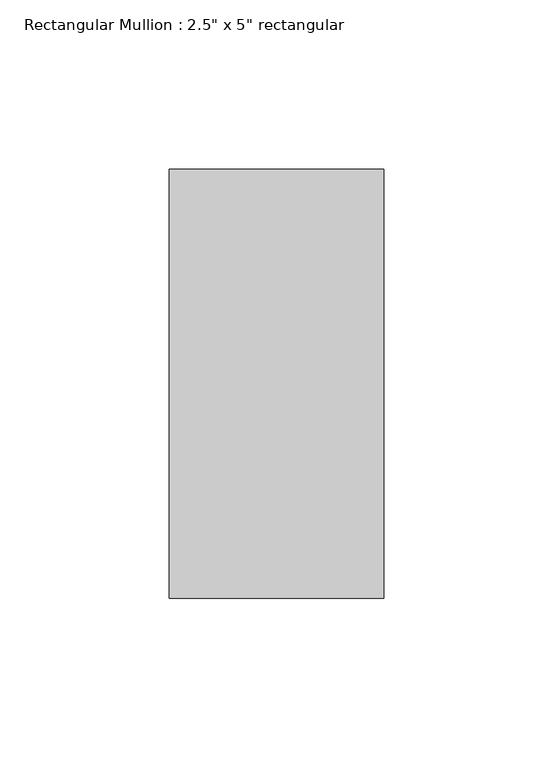
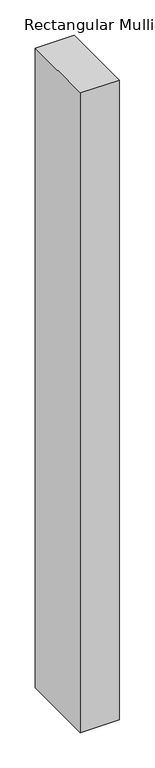
"""IFC4 building model written with IfcOpenShell, lengths in millimetres: member geometry."""

import ifcopenshell
import ifcopenshell.guid

model = None  # the IFC model being written
_history = None  # IfcOwnerHistory: only IFC2X3 demands one
_inside = {}  # id of a spatial element -> (the spatial element, [elements in it])
_under = {}  # id of a project, library or spatial element -> (it, [spatial elements below it])
_declared = {}  # id of a project -> (the project, [libraries it declares])
_typed = {}  # id of a type object -> (the type object, [elements of that type])
_made_of = {}  # id of a material, layer set ... -> (it, [elements and type objects made of it])


def new_model(schema):
    """Start an empty IFC model of exactly this schema.

    Asked for "IFC4X3", IfcOpenShell would pick the latest addendum, in which some entities
    have other attributes; the version numbers below select the first issue.
    IFC2X3 requires an IfcOwnerHistory on every rooted entity: one is made here for all.
    """
    global model, _history
    if schema == "IFC4X3":
        model = ifcopenshell.file(schema_version=(4, 3, 0, 0))
    else:
        model = ifcopenshell.file(schema=schema)
    _inside.clear()
    _under.clear()
    _declared.clear()
    _typed.clear()
    _made_of.clear()
    _history = None
    if model.schema == "IFC2X3":
        org = make("IfcOrganization", Name="unknown")
        user = make(
            "IfcPersonAndOrganization",
            ThePerson=make("IfcPerson", FamilyName="unknown"),
            TheOrganization=org,
        )
        app = make(
            "IfcApplication",
            ApplicationDeveloper=org,
            Version="unknown",
            ApplicationFullName="unknown",
            ApplicationIdentifier="unknown",
        )
        _history = make(
            "IfcOwnerHistory",
            OwningUser=user,
            OwningApplication=app,
            ChangeAction="ADDED",
            CreationDate=0,
        )
    return model


def make(cls, **values):
    """One entity of the class cls with the attributes given. An attribute that is None is left unset."""
    return model.create_entity(
        cls, **{name: value for name, value in values.items() if value is not None}
    )


def rooted(cls, **values):
    """An entity with a GlobalId (a new one), such as an element, a storey or a relation."""
    return make(cls, GlobalId=ifcopenshell.guid.new(), OwnerHistory=_history, **values)


def si_unit(unit_type, name, prefix=None):
    """IfcSIUnit, for example si_unit("LENGTHUNIT", "METRE", prefix="MILLI")."""
    return make("IfcSIUnit", UnitType=unit_type, Prefix=prefix, Name=name)


def assignment(units):
    """IfcUnitAssignment: the units of a project."""
    return None if units is None else make("IfcUnitAssignment", Units=units)


def point(xyz):
    """IfcCartesianPoint."""
    return None if xyz is None else make("IfcCartesianPoint", Coordinates=xyz)


def direction(xyz):
    """IfcDirection."""
    return None if xyz is None else make("IfcDirection", DirectionRatios=xyz)


def frame(location, z_axis=None, x_axis=None):
    """IfcAxis2Placement3D, a coordinate frame: its origin and axes. An axis left out is left unset."""
    return make(
        "IfcAxis2Placement3D",
        Location=point(location),
        Axis=direction(z_axis),
        RefDirection=direction(x_axis),
    )


def origin():
    """The frame at (0, 0, 0) with its axes left unset."""
    return frame((0.0, 0.0, 0.0))


def place(relative_to, where):
    """IfcLocalPlacement: puts the frame where relative to a parent placement (None: the world)."""
    return make(
        "IfcLocalPlacement", PlacementRelTo=relative_to, RelativePlacement=where
    )


def context(
    kind, dimensions, precision=None, world=None, true_north=None, identifier=None
):
    """IfcGeometricRepresentationContext, for example the 3D "Model" context."""
    return make(
        "IfcGeometricRepresentationContext",
        ContextIdentifier=identifier,
        ContextType=kind,
        CoordinateSpaceDimension=dimensions,
        Precision=precision,
        WorldCoordinateSystem=world,
        TrueNorth=true_north,
    )


def project(units=None, contexts=None):
    """IfcProject with its units and contexts."""
    return rooted(
        "IfcProject",
        Name="project",
        RepresentationContexts=contexts,
        UnitsInContext=assignment(units),
    )


def spatial(cls, under=None, at=None, **own):
    """A site, building, storey or space (cls), placed at a placement, below another one or the project."""
    s = rooted(cls, ObjectPlacement=at, **own)
    if under is not None:
        _under.setdefault(under.id(), (under, []))[1].append(s)
    return s


def polyline(points):
    """IfcPolyline through the points."""
    return make("IfcPolyline", Points=[point(p) for p in points])


def outline(outer, holes=None, kind="AREA"):
    """IfcArbitraryClosedProfileDef: a profile drawn as a closed curve; with holes, ...WithVoids."""
    if holes is None:
        return make("IfcArbitraryClosedProfileDef", ProfileType=kind, OuterCurve=outer)
    return make(
        "IfcArbitraryProfileDefWithVoids",
        ProfileType=kind,
        OuterCurve=outer,
        InnerCurves=holes,
    )


def extrude(swept, where, along, depth):
    """IfcExtrudedAreaSolid: the profile swept, set in the frame where, extruded along a direction by depth."""
    return make(
        "IfcExtrudedAreaSolid",
        SweptArea=swept,
        Position=where,
        ExtrudedDirection=direction(along),
        Depth=depth,
    )


def shape(context_of_items, identifier, shape_type, items):
    """IfcShapeRepresentation: the items that make up one representation, for example the "Body"."""
    return make(
        "IfcShapeRepresentation",
        ContextOfItems=context_of_items,
        RepresentationIdentifier=identifier,
        RepresentationType=shape_type,
        Items=items,
    )


def source(mapping_origin, context_of_items, identifier, shape_type, items):
    """IfcRepresentationMap: a shape defined once, which mapped items show again and again."""
    return make(
        "IfcRepresentationMap",
        MappingOrigin=mapping_origin,
        MappedRepresentation=shape(context_of_items, identifier, shape_type, items),
    )


def transform(
    local_origin,
    x_axis=None,
    y_axis=None,
    z_axis=None,
    scale=None,
    scale2=None,
    scale3=None,
    uniform=True,
):
    """IfcCartesianTransformationOperator3D, or its non-uniform kind. x_axis, y_axis, z_axis: its Axis1, 2, 3."""
    if uniform:
        return make(
            "IfcCartesianTransformationOperator3D",
            Axis1=direction(x_axis),
            Axis2=direction(y_axis),
            LocalOrigin=point(local_origin),
            Scale=scale,
            Axis3=direction(z_axis),
        )
    return make(
        "IfcCartesianTransformationOperator3DnonUniform",
        Axis1=direction(x_axis),
        Axis2=direction(y_axis),
        LocalOrigin=point(local_origin),
        Scale=scale,
        Axis3=direction(z_axis),
        Scale2=scale2,
        Scale3=scale3,
    )


def mapped(mapping_source, mapping_target):
    """IfcMappedItem: shows the shape of a source again, moved by a transform."""
    return make(
        "IfcMappedItem", MappingSource=mapping_source, MappingTarget=mapping_target
    )


def made_of(thing, what):
    """Note that an element or type object is made of a material, layer set ...; save() writes the relation."""
    if what is not None:
        _made_of.setdefault(what.id(), (what, []))[1].append(thing)
    return thing


def element(
    cls,
    number,
    at=None,
    inside=None,
    cuts=None,
    type_object=None,
    material=None,
    context=None,
    identifier="Body",
    shape_type=None,
    held_by="IfcProductDefinitionShape",
    body=None,
    shapes=None,
    **own,
):
    """One element of the class cls, such as IfcWall. Its Tag is "e" and its number.

    at: its placement. inside: the storey or other place that contains it. cuts: it is an
    opening in that element (IfcRelVoidsElement). A single representation is given by context,
    identifier, shape_type and body (its items); several are given by shapes. held_by: the class
    of the entity that holds the representations. save() writes the other relations.
    """
    e = rooted(cls, Tag="e%d" % number, ObjectPlacement=at, **own)
    if body is not None:
        shapes = [shape(context, identifier, shape_type, body)]
    if shapes is not None:
        e.Representation = make(held_by, Representations=shapes)
    if inside is not None:
        _inside.setdefault(inside.id(), (inside, []))[1].append(e)
    if cuts is not None:
        rooted(
            "IfcRelVoidsElement", RelatingBuildingElement=cuts, RelatedOpeningElement=e
        )
    if type_object is not None:
        _typed.setdefault(type_object.id(), (type_object, []))[1].append(e)
    return made_of(e, material)


def aggregate(whole, parts):
    """IfcRelAggregates: a whole, such as a stair, and the parts it consists of."""
    return rooted("IfcRelAggregates", RelatingObject=whole, RelatedObjects=parts)


def save(model, path):
    """Write the relations noted so far, then the file.

    IfcRelAggregates (storeys below a building ...), IfcRelContainedInSpatialStructure (elements
    in a storey), IfcRelDefinesByType, IfcRelAssociatesMaterial and IfcRelDeclares: one each for
    every whole, place, type object, material and project.
    """
    for whole, parts in _under.values():
        aggregate(whole, parts)
    for where, things in _inside.values():
        rooted(
            "IfcRelContainedInSpatialStructure",
            RelatedElements=things,
            RelatingStructure=where,
        )
    for kind, things in _typed.values():
        rooted("IfcRelDefinesByType", RelatedObjects=things, RelatingType=kind)
    for what, things in _made_of.values():
        rooted("IfcRelAssociatesMaterial", RelatedObjects=things, RelatingMaterial=what)
    for by, libraries in _declared.values():
        rooted("IfcRelDeclares", RelatingContext=by, RelatedDefinitions=libraries)
    model.write(path)


def member_1f6f54fd(model_context):
    return source(origin(), model_context, "Body", "SweptSolid", [
        extrude(outline(polyline([(0.0, 63.5), (0.0, -63.5), (-63.5, -63.5), (-63.5, 63.5), (0.0, 63.5)])), frame((0.0, 0.0, -1103.9315359), z_axis=(0.0, 0.0, 1.0), x_axis=(1.0, 0.0, 0.0)), (0.0, 0.0, 1.0), 1103.9315359),
    ])


if __name__ == "__main__":
    model = new_model("IFC4")
    model_context = context("Model", 3, world=origin())
    ifc_project = project(units=[si_unit("LENGTHUNIT", "METRE", prefix="MILLI")], contexts=[model_context])
    site = spatial("IfcSite", under=ifc_project)
    building = spatial("IfcBuilding", under=site)
    placement = place(None, origin())
    member_shape = member_1f6f54fd(model_context)
    element("IfcMember", 1, ObjectType="Rectangular Mullion : 2.5\" x 5\" rectangular", at=placement, inside=building, context=model_context, shape_type="MappedRepresentation", body=[
        mapped(member_shape, transform((0.0, 0.0, 0.0), x_axis=(1.0, 0.0, 0.0), y_axis=(0.0, 1.0, 0.0), z_axis=(0.0, 0.0, 1.0))),
    ])
    save(model, "model.ifc")

# Revit data of these elements
# Type "Rectangular Mullion : 2.5\" x 5\" rectangular"
#   built-in parameter 1007304 = 0.416667 (stored number, unit not read)
#   built-in parameter 1007301 = 0.104167 (stored number, unit not read)
#   built-in parameter 1007300 = 0.104167 (stored number, unit not read)
# Element 1 (IfcMember, "Rectangular Mullion : 2.5\" x 5\" rectangular")
#   Materials on its faces: "Aluminum"
# Materials
#   "Aluminum": class "Metal", colour RGB 247 247 247, transparency 0, Description = "Aluminum 6061", Cost = 0
